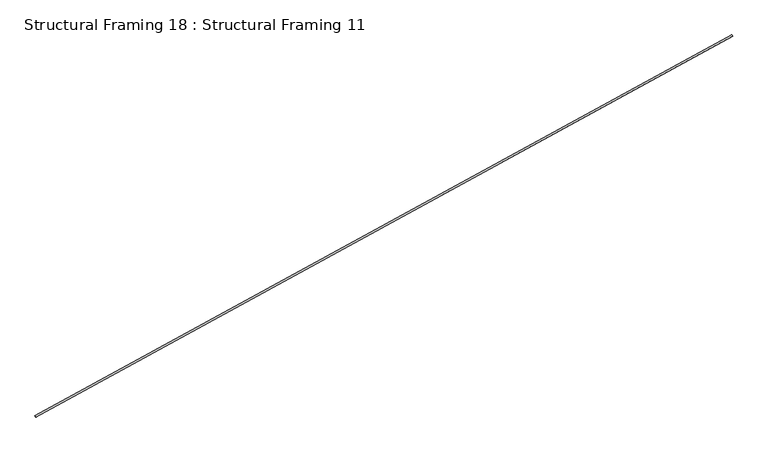
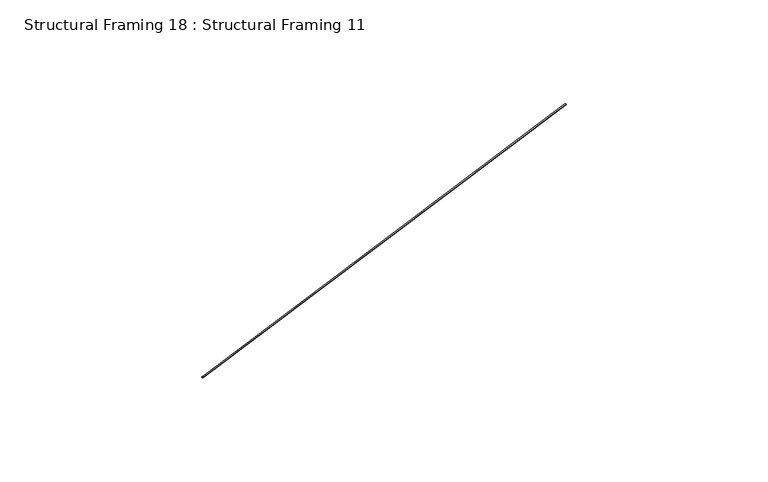
"""IFC4 building model written with IfcOpenShell, lengths in millimetres: beam geometry, Structural Framing 18 : Structural Framing 11."""

import ifcopenshell
import ifcopenshell.guid

model = None  # the IFC model being written
_history = None  # IfcOwnerHistory: only IFC2X3 demands one
_inside = {}  # id of a spatial element -> (the spatial element, [elements in it])
_under = {}  # id of a project, library or spatial element -> (it, [spatial elements below it])
_declared = {}  # id of a project -> (the project, [libraries it declares])
_typed = {}  # id of a type object -> (the type object, [elements of that type])
_made_of = {}  # id of a material, layer set ... -> (it, [elements and type objects made of it])


def new_model(schema):
    """Start an empty IFC model of exactly this schema.

    Asked for "IFC4X3", IfcOpenShell would pick the latest addendum, in which some entities
    have other attributes; the version numbers below select the first issue.
    IFC2X3 requires an IfcOwnerHistory on every rooted entity: one is made here for all.
    """
    global model, _history
    if schema == "IFC4X3":
        model = ifcopenshell.file(schema_version=(4, 3, 0, 0))
    else:
        model = ifcopenshell.file(schema=schema)
    _inside.clear()
    _under.clear()
    _declared.clear()
    _typed.clear()
    _made_of.clear()
    _history = None
    if model.schema == "IFC2X3":
        org = make("IfcOrganization", Name="unknown")
        user = make(
            "IfcPersonAndOrganization",
            ThePerson=make("IfcPerson", FamilyName="unknown"),
            TheOrganization=org,
        )
        app = make(
            "IfcApplication",
            ApplicationDeveloper=org,
            Version="unknown",
            ApplicationFullName="unknown",
            ApplicationIdentifier="unknown",
        )
        _history = make(
            "IfcOwnerHistory",
            OwningUser=user,
            OwningApplication=app,
            ChangeAction="ADDED",
            CreationDate=0,
        )
    return model


def make(cls, **values):
    """One entity of the class cls with the attributes given. An attribute that is None is left unset."""
    return model.create_entity(
        cls, **{name: value for name, value in values.items() if value is not None}
    )


def rooted(cls, **values):
    """An entity with a GlobalId (a new one), such as an element, a storey or a relation."""
    return make(cls, GlobalId=ifcopenshell.guid.new(), OwnerHistory=_history, **values)


def si_unit(unit_type, name, prefix=None):
    """IfcSIUnit, for example si_unit("LENGTHUNIT", "METRE", prefix="MILLI")."""
    return make("IfcSIUnit", UnitType=unit_type, Prefix=prefix, Name=name)


def assignment(units):
    """IfcUnitAssignment: the units of a project."""
    return None if units is None else make("IfcUnitAssignment", Units=units)


def point(xyz):
    """IfcCartesianPoint."""
    return None if xyz is None else make("IfcCartesianPoint", Coordinates=xyz)


def direction(xyz):
    """IfcDirection."""
    return None if xyz is None else make("IfcDirection", DirectionRatios=xyz)


def frame(location, z_axis=None, x_axis=None):
    """IfcAxis2Placement3D, a coordinate frame: its origin and axes. An axis left out is left unset."""
    return make(
        "IfcAxis2Placement3D",
        Location=point(location),
        Axis=direction(z_axis),
        RefDirection=direction(x_axis),
    )


def frame_2d(location, x_axis=None):
    """IfcAxis2Placement2D, a coordinate frame in the plane: its origin and x axis."""
    return make(
        "IfcAxis2Placement2D", Location=point(location), RefDirection=direction(x_axis)
    )


def origin():
    """The frame at (0, 0, 0) with its axes left unset."""
    return frame((0.0, 0.0, 0.0))


def origin_2d():
    """The frame at (0, 0) in the plane with its x axis left unset."""
    return frame_2d((0.0, 0.0))


def place(relative_to, where):
    """IfcLocalPlacement: puts the frame where relative to a parent placement (None: the world)."""
    return make(
        "IfcLocalPlacement", PlacementRelTo=relative_to, RelativePlacement=where
    )


def context(
    kind, dimensions, precision=None, world=None, true_north=None, identifier=None
):
    """IfcGeometricRepresentationContext, for example the 3D "Model" context."""
    return make(
        "IfcGeometricRepresentationContext",
        ContextIdentifier=identifier,
        ContextType=kind,
        CoordinateSpaceDimension=dimensions,
        Precision=precision,
        WorldCoordinateSystem=world,
        TrueNorth=true_north,
    )


def project(units=None, contexts=None):
    """IfcProject with its units and contexts."""
    return rooted(
        "IfcProject",
        Name="project",
        RepresentationContexts=contexts,
        UnitsInContext=assignment(units),
    )


def spatial(cls, under=None, at=None, **own):
    """A site, building, storey or space (cls), placed at a placement, below another one or the project."""
    s = rooted(cls, ObjectPlacement=at, **own)
    if under is not None:
        _under.setdefault(under.id(), (under, []))[1].append(s)
    return s


def circle_curve(where, radius):
    """IfcCircle in the frame where."""
    return make("IfcCircle", Position=where, Radius=radius)


def trimmed(basis, trim1, trim2, sense, master):
    """IfcTrimmedCurve: the piece of a basis curve between two trims."""
    return make(
        "IfcTrimmedCurve",
        BasisCurve=basis,
        Trim1=trim1,
        Trim2=trim2,
        SenseAgreement=sense,
        MasterRepresentation=master,
    )


def segment(curve, same_sense, transition):
    """IfcCompositeCurveSegment."""
    return make(
        "IfcCompositeCurveSegment",
        Transition=transition,
        SameSense=same_sense,
        ParentCurve=curve,
    )


def composite_curve(segments, self_intersect=None):
    """IfcCompositeCurve: segments joined end to end."""
    return make("IfcCompositeCurve", Segments=segments, SelfIntersect=self_intersect)


def outline(outer, holes=None, kind="AREA"):
    """IfcArbitraryClosedProfileDef: a profile drawn as a closed curve; with holes, ...WithVoids."""
    if holes is None:
        return make("IfcArbitraryClosedProfileDef", ProfileType=kind, OuterCurve=outer)
    return make(
        "IfcArbitraryProfileDefWithVoids",
        ProfileType=kind,
        OuterCurve=outer,
        InnerCurves=holes,
    )


def extrude(swept, where, along, depth):
    """IfcExtrudedAreaSolid: the profile swept, set in the frame where, extruded along a direction by depth."""
    return make(
        "IfcExtrudedAreaSolid",
        SweptArea=swept,
        Position=where,
        ExtrudedDirection=direction(along),
        Depth=depth,
    )


def shape(context_of_items, identifier, shape_type, items):
    """IfcShapeRepresentation: the items that make up one representation, for example the "Body"."""
    return make(
        "IfcShapeRepresentation",
        ContextOfItems=context_of_items,
        RepresentationIdentifier=identifier,
        RepresentationType=shape_type,
        Items=items,
    )


def source(mapping_origin, context_of_items, identifier, shape_type, items):
    """IfcRepresentationMap: a shape defined once, which mapped items show again and again."""
    return make(
        "IfcRepresentationMap",
        MappingOrigin=mapping_origin,
        MappedRepresentation=shape(context_of_items, identifier, shape_type, items),
    )


def transform(
    local_origin,
    x_axis=None,
    y_axis=None,
    z_axis=None,
    scale=None,
    scale2=None,
    scale3=None,
    uniform=True,
):
    """IfcCartesianTransformationOperator3D, or its non-uniform kind. x_axis, y_axis, z_axis: its Axis1, 2, 3."""
    if uniform:
        return make(
            "IfcCartesianTransformationOperator3D",
            Axis1=direction(x_axis),
            Axis2=direction(y_axis),
            LocalOrigin=point(local_origin),
            Scale=scale,
            Axis3=direction(z_axis),
        )
    return make(
        "IfcCartesianTransformationOperator3DnonUniform",
        Axis1=direction(x_axis),
        Axis2=direction(y_axis),
        LocalOrigin=point(local_origin),
        Scale=scale,
        Axis3=direction(z_axis),
        Scale2=scale2,
        Scale3=scale3,
    )


def mapped(mapping_source, mapping_target):
    """IfcMappedItem: shows the shape of a source again, moved by a transform."""
    return make(
        "IfcMappedItem", MappingSource=mapping_source, MappingTarget=mapping_target
    )


def made_of(thing, what):
    """Note that an element or type object is made of a material, layer set ...; save() writes the relation."""
    if what is not None:
        _made_of.setdefault(what.id(), (what, []))[1].append(thing)
    return thing


def element(
    cls,
    number,
    at=None,
    inside=None,
    cuts=None,
    type_object=None,
    material=None,
    context=None,
    identifier="Body",
    shape_type=None,
    held_by="IfcProductDefinitionShape",
    body=None,
    shapes=None,
    **own,
):
    """One element of the class cls, such as IfcWall. Its Tag is "e" and its number.

    at: its placement. inside: the storey or other place that contains it. cuts: it is an
    opening in that element (IfcRelVoidsElement). A single representation is given by context,
    identifier, shape_type and body (its items); several are given by shapes. held_by: the class
    of the entity that holds the representations. save() writes the other relations.
    """
    e = rooted(cls, Tag="e%d" % number, ObjectPlacement=at, **own)
    if body is not None:
        shapes = [shape(context, identifier, shape_type, body)]
    if shapes is not None:
        e.Representation = make(held_by, Representations=shapes)
    if inside is not None:
        _inside.setdefault(inside.id(), (inside, []))[1].append(e)
    if cuts is not None:
        rooted(
            "IfcRelVoidsElement", RelatingBuildingElement=cuts, RelatedOpeningElement=e
        )
    if type_object is not None:
        _typed.setdefault(type_object.id(), (type_object, []))[1].append(e)
    return made_of(e, material)


def aggregate(whole, parts):
    """IfcRelAggregates: a whole, such as a stair, and the parts it consists of."""
    return rooted("IfcRelAggregates", RelatingObject=whole, RelatedObjects=parts)


def save(model, path):
    """Write the relations noted so far, then the file.

    IfcRelAggregates (storeys below a building ...), IfcRelContainedInSpatialStructure (elements
    in a storey), IfcRelDefinesByType, IfcRelAssociatesMaterial and IfcRelDeclares: one each for
    every whole, place, type object, material and project.
    """
    for whole, parts in _under.values():
        aggregate(whole, parts)
    for where, things in _inside.values():
        rooted(
            "IfcRelContainedInSpatialStructure",
            RelatedElements=things,
            RelatingStructure=where,
        )
    for kind, things in _typed.values():
        rooted("IfcRelDefinesByType", RelatedObjects=things, RelatingType=kind)
    for what, things in _made_of.values():
        rooted("IfcRelAssociatesMaterial", RelatedObjects=things, RelatingMaterial=what)
    for by, libraries in _declared.values():
        rooted("IfcRelDeclares", RelatingContext=by, RelatedDefinitions=libraries)
    model.write(path)


def structural_framing_18_structural_framing_11_23cca81f(model_context):
    return source(origin(), model_context, "Body", "SweptSolid", [
        extrude(outline(composite_curve([segment(trimmed(circle_curve(origin_2d(), 6.35), [point((0.0, 6.35))], [point((0.0, -6.3499999))], False, "CARTESIAN"), True, "CONTINUOUS"), segment(trimmed(circle_curve(origin_2d(), 6.35), [point((0.0, -6.3499999))], [point((0.0, 6.35))], False, "CARTESIAN"), True, "CONTINUOUS")], self_intersect=False)), frame((17939.5405771, 10048.6776702, 4933.3856456), z_axis=(-0.8714985593718723, -0.47575600371495647, 0.11893900092873574), x_axis=(0.0, 0.24253562503632659, 0.9701425001453335)), (0.0, 0.0, 1.0), 6120.4961437),
    ])


if __name__ == "__main__":
    model = new_model("IFC4")
    model_context = context("Model", 3, world=origin())
    ifc_project = project(units=[si_unit("LENGTHUNIT", "METRE", prefix="MILLI")], contexts=[model_context])
    site = spatial("IfcSite", under=ifc_project)
    building = spatial("IfcBuilding", under=site)
    placement = place(None, origin())
    structural_framing_18_structural_framing_11_shape = structural_framing_18_structural_framing_11_23cca81f(model_context)
    element("IfcBeam", 1, ObjectType="Structural Framing 18 : Structural Framing 11", at=placement, inside=building, context=model_context, shape_type="MappedRepresentation", body=[
        mapped(structural_framing_18_structural_framing_11_shape, transform((0.0, 0.0, 0.0), x_axis=(1.0, 0.0, 0.0), y_axis=(0.0, 1.0, 0.0), z_axis=(0.0, 0.0, 1.0))),
    ])
    save(model, "model.ifc")

# Revit data of these elements
# Type "Structural Framing 18 : Structural Framing 11"
#   Structural Material [instance default] = EXISTING LATERAL BRACING (1/4" CABLE)
# Element 1 (IfcBeam, "Structural Framing 18 : Structural Framing 11")
#   Materials on its faces: "EXISTING LATERAL BRACING (1/4\" CABLE)"
# Materials
#   "EXISTING LATERAL BRACING (1/4\" CABLE)": class "Generic", colour RGB 120 120 120, transparency 0, Cost = 0
